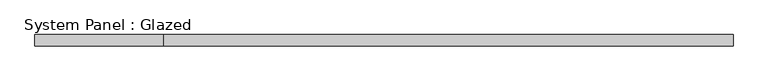
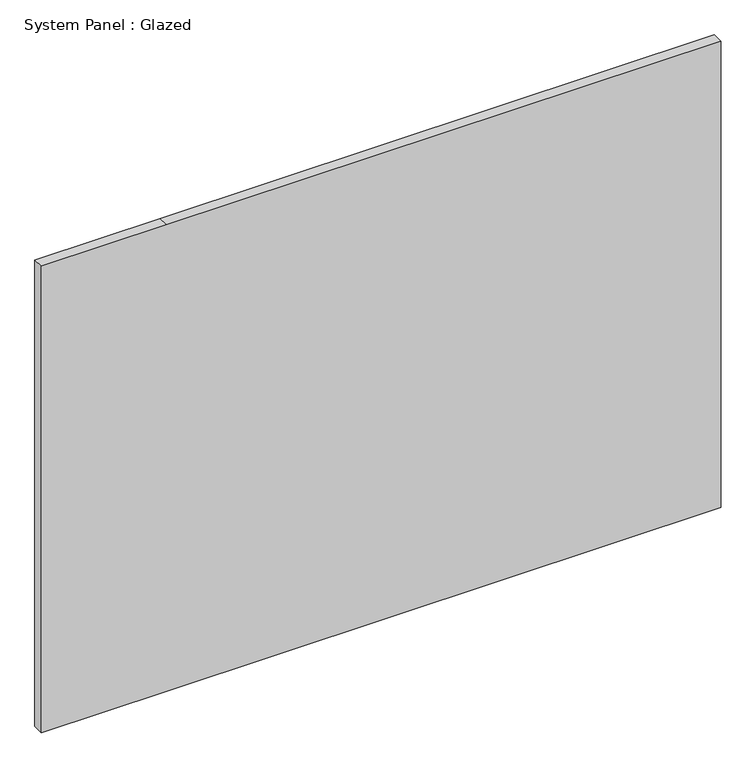
"""IFC4 building model written with IfcOpenShell, lengths in millimetres: plate geometry, System Panel : Glazed."""

import ifcopenshell
import ifcopenshell.guid

model = None  # the IFC model being written
_history = None  # IfcOwnerHistory: only IFC2X3 demands one
_inside = {}  # id of a spatial element -> (the spatial element, [elements in it])
_under = {}  # id of a project, library or spatial element -> (it, [spatial elements below it])
_declared = {}  # id of a project -> (the project, [libraries it declares])
_typed = {}  # id of a type object -> (the type object, [elements of that type])
_made_of = {}  # id of a material, layer set ... -> (it, [elements and type objects made of it])


def new_model(schema):
    """Start an empty IFC model of exactly this schema.

    Asked for "IFC4X3", IfcOpenShell would pick the latest addendum, in which some entities
    have other attributes; the version numbers below select the first issue.
    IFC2X3 requires an IfcOwnerHistory on every rooted entity: one is made here for all.
    """
    global model, _history
    if schema == "IFC4X3":
        model = ifcopenshell.file(schema_version=(4, 3, 0, 0))
    else:
        model = ifcopenshell.file(schema=schema)
    _inside.clear()
    _under.clear()
    _declared.clear()
    _typed.clear()
    _made_of.clear()
    _history = None
    if model.schema == "IFC2X3":
        org = make("IfcOrganization", Name="unknown")
        user = make(
            "IfcPersonAndOrganization",
            ThePerson=make("IfcPerson", FamilyName="unknown"),
            TheOrganization=org,
        )
        app = make(
            "IfcApplication",
            ApplicationDeveloper=org,
            Version="unknown",
            ApplicationFullName="unknown",
            ApplicationIdentifier="unknown",
        )
        _history = make(
            "IfcOwnerHistory",
            OwningUser=user,
            OwningApplication=app,
            ChangeAction="ADDED",
            CreationDate=0,
        )
    return model


def make(cls, **values):
    """One entity of the class cls with the attributes given. An attribute that is None is left unset."""
    return model.create_entity(
        cls, **{name: value for name, value in values.items() if value is not None}
    )


def rooted(cls, **values):
    """An entity with a GlobalId (a new one), such as an element, a storey or a relation."""
    return make(cls, GlobalId=ifcopenshell.guid.new(), OwnerHistory=_history, **values)


def si_unit(unit_type, name, prefix=None):
    """IfcSIUnit, for example si_unit("LENGTHUNIT", "METRE", prefix="MILLI")."""
    return make("IfcSIUnit", UnitType=unit_type, Prefix=prefix, Name=name)


def assignment(units):
    """IfcUnitAssignment: the units of a project."""
    return None if units is None else make("IfcUnitAssignment", Units=units)


def point(xyz):
    """IfcCartesianPoint."""
    return None if xyz is None else make("IfcCartesianPoint", Coordinates=xyz)


def direction(xyz):
    """IfcDirection."""
    return None if xyz is None else make("IfcDirection", DirectionRatios=xyz)


def frame(location, z_axis=None, x_axis=None):
    """IfcAxis2Placement3D, a coordinate frame: its origin and axes. An axis left out is left unset."""
    return make(
        "IfcAxis2Placement3D",
        Location=point(location),
        Axis=direction(z_axis),
        RefDirection=direction(x_axis),
    )


def origin():
    """The frame at (0, 0, 0) with its axes left unset."""
    return frame((0.0, 0.0, 0.0))


def place(relative_to, where):
    """IfcLocalPlacement: puts the frame where relative to a parent placement (None: the world)."""
    return make(
        "IfcLocalPlacement", PlacementRelTo=relative_to, RelativePlacement=where
    )


def context(
    kind, dimensions, precision=None, world=None, true_north=None, identifier=None
):
    """IfcGeometricRepresentationContext, for example the 3D "Model" context."""
    return make(
        "IfcGeometricRepresentationContext",
        ContextIdentifier=identifier,
        ContextType=kind,
        CoordinateSpaceDimension=dimensions,
        Precision=precision,
        WorldCoordinateSystem=world,
        TrueNorth=true_north,
    )


def project(units=None, contexts=None):
    """IfcProject with its units and contexts."""
    return rooted(
        "IfcProject",
        Name="project",
        RepresentationContexts=contexts,
        UnitsInContext=assignment(units),
    )


def spatial(cls, under=None, at=None, **own):
    """A site, building, storey or space (cls), placed at a placement, below another one or the project."""
    s = rooted(cls, ObjectPlacement=at, **own)
    if under is not None:
        _under.setdefault(under.id(), (under, []))[1].append(s)
    return s


def polyline(points):
    """IfcPolyline through the points."""
    return make("IfcPolyline", Points=[point(p) for p in points])


def outline(outer, holes=None, kind="AREA"):
    """IfcArbitraryClosedProfileDef: a profile drawn as a closed curve; with holes, ...WithVoids."""
    if holes is None:
        return make("IfcArbitraryClosedProfileDef", ProfileType=kind, OuterCurve=outer)
    return make(
        "IfcArbitraryProfileDefWithVoids",
        ProfileType=kind,
        OuterCurve=outer,
        InnerCurves=holes,
    )


def extrude(swept, where, along, depth):
    """IfcExtrudedAreaSolid: the profile swept, set in the frame where, extruded along a direction by depth."""
    return make(
        "IfcExtrudedAreaSolid",
        SweptArea=swept,
        Position=where,
        ExtrudedDirection=direction(along),
        Depth=depth,
    )


def shape(context_of_items, identifier, shape_type, items):
    """IfcShapeRepresentation: the items that make up one representation, for example the "Body"."""
    return make(
        "IfcShapeRepresentation",
        ContextOfItems=context_of_items,
        RepresentationIdentifier=identifier,
        RepresentationType=shape_type,
        Items=items,
    )


def source(mapping_origin, context_of_items, identifier, shape_type, items):
    """IfcRepresentationMap: a shape defined once, which mapped items show again and again."""
    return make(
        "IfcRepresentationMap",
        MappingOrigin=mapping_origin,
        MappedRepresentation=shape(context_of_items, identifier, shape_type, items),
    )


def transform(
    local_origin,
    x_axis=None,
    y_axis=None,
    z_axis=None,
    scale=None,
    scale2=None,
    scale3=None,
    uniform=True,
):
    """IfcCartesianTransformationOperator3D, or its non-uniform kind. x_axis, y_axis, z_axis: its Axis1, 2, 3."""
    if uniform:
        return make(
            "IfcCartesianTransformationOperator3D",
            Axis1=direction(x_axis),
            Axis2=direction(y_axis),
            LocalOrigin=point(local_origin),
            Scale=scale,
            Axis3=direction(z_axis),
        )
    return make(
        "IfcCartesianTransformationOperator3DnonUniform",
        Axis1=direction(x_axis),
        Axis2=direction(y_axis),
        LocalOrigin=point(local_origin),
        Scale=scale,
        Axis3=direction(z_axis),
        Scale2=scale2,
        Scale3=scale3,
    )


def mapped(mapping_source, mapping_target):
    """IfcMappedItem: shows the shape of a source again, moved by a transform."""
    return make(
        "IfcMappedItem", MappingSource=mapping_source, MappingTarget=mapping_target
    )


def made_of(thing, what):
    """Note that an element or type object is made of a material, layer set ...; save() writes the relation."""
    if what is not None:
        _made_of.setdefault(what.id(), (what, []))[1].append(thing)
    return thing


def element(
    cls,
    number,
    at=None,
    inside=None,
    cuts=None,
    type_object=None,
    material=None,
    context=None,
    identifier="Body",
    shape_type=None,
    held_by="IfcProductDefinitionShape",
    body=None,
    shapes=None,
    **own,
):
    """One element of the class cls, such as IfcWall. Its Tag is "e" and its number.

    at: its placement. inside: the storey or other place that contains it. cuts: it is an
    opening in that element (IfcRelVoidsElement). A single representation is given by context,
    identifier, shape_type and body (its items); several are given by shapes. held_by: the class
    of the entity that holds the representations. save() writes the other relations.
    """
    e = rooted(cls, Tag="e%d" % number, ObjectPlacement=at, **own)
    if body is not None:
        shapes = [shape(context, identifier, shape_type, body)]
    if shapes is not None:
        e.Representation = make(held_by, Representations=shapes)
    if inside is not None:
        _inside.setdefault(inside.id(), (inside, []))[1].append(e)
    if cuts is not None:
        rooted(
            "IfcRelVoidsElement", RelatingBuildingElement=cuts, RelatedOpeningElement=e
        )
    if type_object is not None:
        _typed.setdefault(type_object.id(), (type_object, []))[1].append(e)
    return made_of(e, material)


def aggregate(whole, parts):
    """IfcRelAggregates: a whole, such as a stair, and the parts it consists of."""
    return rooted("IfcRelAggregates", RelatingObject=whole, RelatedObjects=parts)


def save(model, path):
    """Write the relations noted so far, then the file.

    IfcRelAggregates (storeys below a building ...), IfcRelContainedInSpatialStructure (elements
    in a storey), IfcRelDefinesByType, IfcRelAssociatesMaterial and IfcRelDeclares: one each for
    every whole, place, type object, material and project.
    """
    for whole, parts in _under.values():
        aggregate(whole, parts)
    for where, things in _inside.values():
        rooted(
            "IfcRelContainedInSpatialStructure",
            RelatedElements=things,
            RelatingStructure=where,
        )
    for kind, things in _typed.values():
        rooted("IfcRelDefinesByType", RelatedObjects=things, RelatingType=kind)
    for what, things in _made_of.values():
        rooted("IfcRelAssociatesMaterial", RelatedObjects=things, RelatingMaterial=what)
    for by, libraries in _declared.values():
        rooted("IfcRelDeclares", RelatingContext=by, RelatedDefinitions=libraries)
    model.write(path)


def system_panel_glazed_835a6d4f(model_context):
    return source(origin(), model_context, "Body", "SweptSolid", [
        extrude(outline(polyline([(0.0, -774.7), (0.0, -488.95), (0.0, 774.7), (1123.95, 774.7), (1123.95, -488.95), (1123.95, -774.7), (0.0, -774.7)])), frame((0.0, 19.05, 0.0), z_axis=(0.0, 1.0, 0.0), x_axis=(0.0, 0.0, 1.0)), (0.0, 0.0, 1.0), 25.4),
    ])


if __name__ == "__main__":
    model = new_model("IFC4")
    model_context = context("Model", 3, world=origin())
    ifc_project = project(units=[si_unit("LENGTHUNIT", "METRE", prefix="MILLI")], contexts=[model_context])
    site = spatial("IfcSite", under=ifc_project)
    building = spatial("IfcBuilding", under=site)
    placement = place(None, origin())
    system_panel_glazed_shape = system_panel_glazed_835a6d4f(model_context)
    element("IfcPlate", 1, ObjectType="System Panel : Glazed", at=placement, inside=building, context=model_context, shape_type="MappedRepresentation", body=[
        mapped(system_panel_glazed_shape, transform((0.0, 0.0, 0.0), x_axis=(1.0, 0.0, 0.0), y_axis=(0.0, 1.0, 0.0), z_axis=(0.0, 0.0, 1.0))),
    ])
    save(model, "model.ifc")

# Revit data of these elements
# Element 1 (IfcPlate, "System Panel : Glazed")
#   Materials on its faces: "Glass"
# Materials
#   "Glass": class "Glass", colour RGB 0 128 192, transparency 0.75
